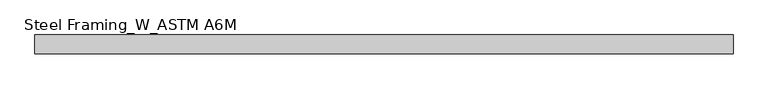
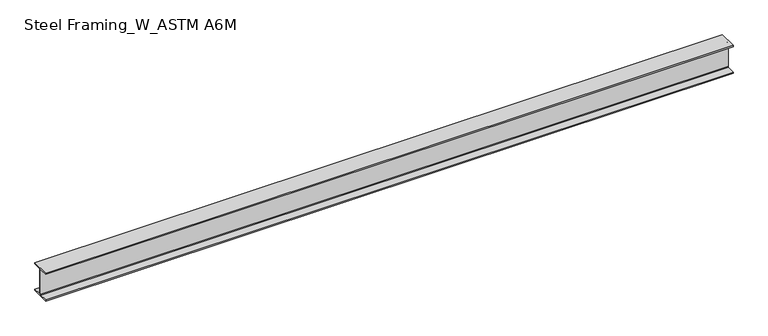
"""IFC4 building model written with IfcOpenShell, lengths in millimetres: beam geometry, Steel Framing_W_ASTM A6M : H_SB_AR_S02_W410x114_B9."""

from ifc_helpers import new_model, si_unit, point, frame, frame_2d, origin, place, context, project, spatial, polyline, circle_curve, trimmed, segment, composite_curve, outline, extrude, source, transform, mapped, element, save


def steel_framing_w_astm_a6m_4c16a149(model_context):
    return source(origin(), model_context, "Body", "SweptSolid", [
        extrude(outline(composite_curve([segment(polyline([(131.0, -190.2), (131.0, -209.5), (-131.0, -209.5), (-131.0, -190.2), (-16.0, -190.2)]), True, "CONTINUOUS"), segment(trimmed(circle_curve(frame_2d((-16.0, -180.0)), 10.2), [point((-16.0, -190.2))], [point((-5.8, -180.0))], True, "CARTESIAN"), True, "CONTINUOUS"), segment(polyline([(-5.8, -180.0), (-5.8, 180.0)]), True, "CONTINUOUS"), segment(trimmed(circle_curve(frame_2d((-16.0, 180.0)), 10.2), [point((-5.8, 180.0))], [point((-16.0, 190.2))], True, "CARTESIAN"), True, "CONTINUOUS"), segment(polyline([(-16.0, 190.2), (-131.0, 190.2), (-131.0, 209.5), (131.0, 209.5), (131.0, 190.2), (16.0, 190.2)]), True, "CONTINUOUS"), segment(trimmed(circle_curve(frame_2d((16.0, 180.0)), 10.2), [point((16.0, 190.2))], [point((5.8, 180.0))], True, "CARTESIAN"), True, "CONTINUOUS"), segment(polyline([(5.8, 180.0), (5.8, -180.0)]), True, "CONTINUOUS"), segment(trimmed(circle_curve(frame_2d((16.0, -180.0)), 10.2), [point((5.8, -180.0))], [point((16.0, -190.2))], True, "CARTESIAN"), True, "CONTINUOUS"), segment(polyline([(16.0, -190.2), (131.0, -190.2)]), True, "CONTINUOUS")], self_intersect=False)), frame((-4885.8, 0.0, 0.0), z_axis=(1.0, 0.0, 0.0), x_axis=(0.0, 1.0, 0.0)), (0.0, 0.0, 1.0), 9771.6),
    ])


if __name__ == "__main__":
    model = new_model("IFC4")
    model_context = context("Model", 3, world=origin())
    ifc_project = project(units=[si_unit("LENGTHUNIT", "METRE", prefix="MILLI")], contexts=[model_context])
    site = spatial("IfcSite", under=ifc_project)
    building = spatial("IfcBuilding", under=site)
    placement = place(None, origin())
    steel_framing_w_astm_a6m_shape = steel_framing_w_astm_a6m_4c16a149(model_context)
    element("IfcBeam", 1, ObjectType="Steel Framing_W_ASTM A6M : H_SB_AR_S02_W410x114_B9", at=placement, inside=building, context=model_context, shape_type="MappedRepresentation", body=[
        mapped(steel_framing_w_astm_a6m_shape, transform((0.0, 0.0, 0.0), x_axis=(1.0, 0.0, 0.0), y_axis=(0.0, 1.0, 0.0), z_axis=(0.0, 0.0, 1.0))),
    ])
    save(model, "model.ifc")

# Revit data of these elements
# Type "Steel Framing_W_ASTM A6M : H_SB_AR_S02_W410x114_B9"
#   Section Name Key = "W16x77"
#   Width = 26.2 cm
#   Web Thickness = 1.16 cm
#   Web Fillet = 1.02 cm
#   Warping Constant = 2310000.0 cm⁶
#   Torsional Moment of Inertia = 149.00 cm⁴
#   Section Area = 146.0 cm²
#   Plastic Modulus weak axis = 674.0 cm³
#   Plastic Modulus strong axis = 2460.0 cm³
#   Perimeter = 1.84 m²/m
#   Nominal Weight = 114.00 kgf/m
#   Moment of Inertia weak axis = 5740.00 cm⁴
#   Moment of Inertia strong axis = 46200.00 cm⁴
#   Height = 41.9 cm
#   Flange Thickness = 1.93 cm
#   Elastic Modulus weak axis = 441.0 cm³
#   Elastic Modulus strong axis = 2200.0 cm³
#   Centroid Vertical = 20.95 cm
#   Centroid Horizontal = 13.1 cm
#   Length [instance default] = 1500 mm
#   Structural Material [instance default] = Steel, 45-345
#   Bolt Spacing = 0
#   Assembly Code = ""
# Element 1 (IfcBeam, "Steel Framing_W_ASTM A6M : H_SB_AR_S02_W410x114_B9")
#   Materials on its faces: "Steel, 45-345"
# Materials
#   "Steel, 45-345": class "Metal", colour RGB 189 187 185, transparency 0, Description = "Steel 345 MPa", Cost = 0
